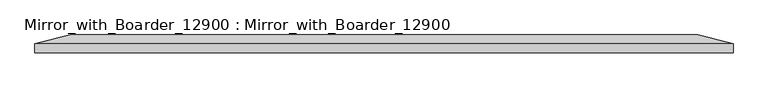
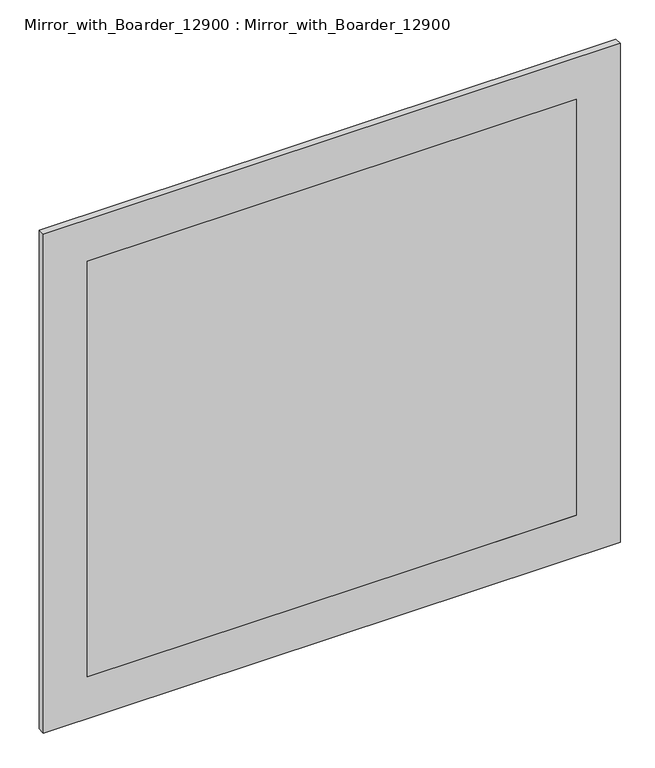
"""IFC4 building model written with IfcOpenShell, lengths in millimetres: proxy geometry, Mirror_with_Boarder_12900 : Mirror_with_Boarder_12900."""

import ifcopenshell
import ifcopenshell.guid

model = None  # the IFC model being written
_history = None  # IfcOwnerHistory: only IFC2X3 demands one
_inside = {}  # id of a spatial element -> (the spatial element, [elements in it])
_under = {}  # id of a project, library or spatial element -> (it, [spatial elements below it])
_declared = {}  # id of a project -> (the project, [libraries it declares])
_typed = {}  # id of a type object -> (the type object, [elements of that type])
_made_of = {}  # id of a material, layer set ... -> (it, [elements and type objects made of it])


def new_model(schema):
    """Start an empty IFC model of exactly this schema.

    Asked for "IFC4X3", IfcOpenShell would pick the latest addendum, in which some entities
    have other attributes; the version numbers below select the first issue.
    IFC2X3 requires an IfcOwnerHistory on every rooted entity: one is made here for all.
    """
    global model, _history
    if schema == "IFC4X3":
        model = ifcopenshell.file(schema_version=(4, 3, 0, 0))
    else:
        model = ifcopenshell.file(schema=schema)
    _inside.clear()
    _under.clear()
    _declared.clear()
    _typed.clear()
    _made_of.clear()
    _history = None
    if model.schema == "IFC2X3":
        org = make("IfcOrganization", Name="unknown")
        user = make(
            "IfcPersonAndOrganization",
            ThePerson=make("IfcPerson", FamilyName="unknown"),
            TheOrganization=org,
        )
        app = make(
            "IfcApplication",
            ApplicationDeveloper=org,
            Version="unknown",
            ApplicationFullName="unknown",
            ApplicationIdentifier="unknown",
        )
        _history = make(
            "IfcOwnerHistory",
            OwningUser=user,
            OwningApplication=app,
            ChangeAction="ADDED",
            CreationDate=0,
        )
    return model


def make(cls, **values):
    """One entity of the class cls with the attributes given. An attribute that is None is left unset."""
    return model.create_entity(
        cls, **{name: value for name, value in values.items() if value is not None}
    )


def rooted(cls, **values):
    """An entity with a GlobalId (a new one), such as an element, a storey or a relation."""
    return make(cls, GlobalId=ifcopenshell.guid.new(), OwnerHistory=_history, **values)


def si_unit(unit_type, name, prefix=None):
    """IfcSIUnit, for example si_unit("LENGTHUNIT", "METRE", prefix="MILLI")."""
    return make("IfcSIUnit", UnitType=unit_type, Prefix=prefix, Name=name)


def assignment(units):
    """IfcUnitAssignment: the units of a project."""
    return None if units is None else make("IfcUnitAssignment", Units=units)


def point(xyz):
    """IfcCartesianPoint."""
    return None if xyz is None else make("IfcCartesianPoint", Coordinates=xyz)


def direction(xyz):
    """IfcDirection."""
    return None if xyz is None else make("IfcDirection", DirectionRatios=xyz)


def frame(location, z_axis=None, x_axis=None):
    """IfcAxis2Placement3D, a coordinate frame: its origin and axes. An axis left out is left unset."""
    return make(
        "IfcAxis2Placement3D",
        Location=point(location),
        Axis=direction(z_axis),
        RefDirection=direction(x_axis),
    )


def origin():
    """The frame at (0, 0, 0) with its axes left unset."""
    return frame((0.0, 0.0, 0.0))


def place(relative_to, where):
    """IfcLocalPlacement: puts the frame where relative to a parent placement (None: the world)."""
    return make(
        "IfcLocalPlacement", PlacementRelTo=relative_to, RelativePlacement=where
    )


def context(
    kind, dimensions, precision=None, world=None, true_north=None, identifier=None
):
    """IfcGeometricRepresentationContext, for example the 3D "Model" context."""
    return make(
        "IfcGeometricRepresentationContext",
        ContextIdentifier=identifier,
        ContextType=kind,
        CoordinateSpaceDimension=dimensions,
        Precision=precision,
        WorldCoordinateSystem=world,
        TrueNorth=true_north,
    )


def project(units=None, contexts=None):
    """IfcProject with its units and contexts."""
    return rooted(
        "IfcProject",
        Name="project",
        RepresentationContexts=contexts,
        UnitsInContext=assignment(units),
    )


def spatial(cls, under=None, at=None, **own):
    """A site, building, storey or space (cls), placed at a placement, below another one or the project."""
    s = rooted(cls, ObjectPlacement=at, **own)
    if under is not None:
        _under.setdefault(under.id(), (under, []))[1].append(s)
    return s


def polyline(points):
    """IfcPolyline through the points."""
    return make("IfcPolyline", Points=[point(p) for p in points])


def outline(outer, holes=None, kind="AREA"):
    """IfcArbitraryClosedProfileDef: a profile drawn as a closed curve; with holes, ...WithVoids."""
    if holes is None:
        return make("IfcArbitraryClosedProfileDef", ProfileType=kind, OuterCurve=outer)
    return make(
        "IfcArbitraryProfileDefWithVoids",
        ProfileType=kind,
        OuterCurve=outer,
        InnerCurves=holes,
    )


def extrude(swept, where, along, depth):
    """IfcExtrudedAreaSolid: the profile swept, set in the frame where, extruded along a direction by depth."""
    return make(
        "IfcExtrudedAreaSolid",
        SweptArea=swept,
        Position=where,
        ExtrudedDirection=direction(along),
        Depth=depth,
    )


def faces_of(points, faces, orient=None, outer=None):
    """IfcFace entities. A face is a list of loops; a loop is a list of indices into points, from 0.

    orient and outer hold one flag for each loop. By default every Orientation is true, the
    first loop of a face is its IfcFaceOuterBound and the others are IfcFaceBound.
    """
    made = []
    for i, loops in enumerate(faces):
        bounds = []
        for j, loop in enumerate(loops):
            is_outer = j == 0 if outer is None else outer[i][j]
            bounds.append(
                make(
                    "IfcFaceOuterBound" if is_outer else "IfcFaceBound",
                    Bound=make("IfcPolyLoop", Polygon=[points[k] for k in loop]),
                    Orientation=True if orient is None else orient[i][j],
                )
            )
        made.append(make("IfcFace", Bounds=bounds))
    return made


def faceted_brep(points, faces, orient=None, outer=None, voids=None):
    """IfcFacetedBrep: a solid bounded by flat faces; with voids (closed shells), ...WithVoids."""
    shared = [point(p) for p in points]
    hull = make("IfcClosedShell", CfsFaces=faces_of(shared, faces, orient, outer))
    if voids is None:
        return make("IfcFacetedBrep", Outer=hull)
    return make(
        "IfcFacetedBrepWithVoids",
        Outer=hull,
        Voids=[
            make(cls, CfsFaces=faces_of(shared, fs, o, b)) for cls, fs, o, b in voids
        ],
    )


def shape(context_of_items, identifier, shape_type, items):
    """IfcShapeRepresentation: the items that make up one representation, for example the "Body"."""
    return make(
        "IfcShapeRepresentation",
        ContextOfItems=context_of_items,
        RepresentationIdentifier=identifier,
        RepresentationType=shape_type,
        Items=items,
    )


def source(mapping_origin, context_of_items, identifier, shape_type, items):
    """IfcRepresentationMap: a shape defined once, which mapped items show again and again."""
    return make(
        "IfcRepresentationMap",
        MappingOrigin=mapping_origin,
        MappedRepresentation=shape(context_of_items, identifier, shape_type, items),
    )


def transform(
    local_origin,
    x_axis=None,
    y_axis=None,
    z_axis=None,
    scale=None,
    scale2=None,
    scale3=None,
    uniform=True,
):
    """IfcCartesianTransformationOperator3D, or its non-uniform kind. x_axis, y_axis, z_axis: its Axis1, 2, 3."""
    if uniform:
        return make(
            "IfcCartesianTransformationOperator3D",
            Axis1=direction(x_axis),
            Axis2=direction(y_axis),
            LocalOrigin=point(local_origin),
            Scale=scale,
            Axis3=direction(z_axis),
        )
    return make(
        "IfcCartesianTransformationOperator3DnonUniform",
        Axis1=direction(x_axis),
        Axis2=direction(y_axis),
        LocalOrigin=point(local_origin),
        Scale=scale,
        Axis3=direction(z_axis),
        Scale2=scale2,
        Scale3=scale3,
    )


def mapped(mapping_source, mapping_target):
    """IfcMappedItem: shows the shape of a source again, moved by a transform."""
    return make(
        "IfcMappedItem", MappingSource=mapping_source, MappingTarget=mapping_target
    )


def made_of(thing, what):
    """Note that an element or type object is made of a material, layer set ...; save() writes the relation."""
    if what is not None:
        _made_of.setdefault(what.id(), (what, []))[1].append(thing)
    return thing


def element(
    cls,
    number,
    at=None,
    inside=None,
    cuts=None,
    type_object=None,
    material=None,
    context=None,
    identifier="Body",
    shape_type=None,
    held_by="IfcProductDefinitionShape",
    body=None,
    shapes=None,
    **own,
):
    """One element of the class cls, such as IfcWall. Its Tag is "e" and its number.

    at: its placement. inside: the storey or other place that contains it. cuts: it is an
    opening in that element (IfcRelVoidsElement). A single representation is given by context,
    identifier, shape_type and body (its items); several are given by shapes. held_by: the class
    of the entity that holds the representations. save() writes the other relations.
    """
    e = rooted(cls, Tag="e%d" % number, ObjectPlacement=at, **own)
    if body is not None:
        shapes = [shape(context, identifier, shape_type, body)]
    if shapes is not None:
        e.Representation = make(held_by, Representations=shapes)
    if inside is not None:
        _inside.setdefault(inside.id(), (inside, []))[1].append(e)
    if cuts is not None:
        rooted(
            "IfcRelVoidsElement", RelatingBuildingElement=cuts, RelatedOpeningElement=e
        )
    if type_object is not None:
        _typed.setdefault(type_object.id(), (type_object, []))[1].append(e)
    return made_of(e, material)


def aggregate(whole, parts):
    """IfcRelAggregates: a whole, such as a stair, and the parts it consists of."""
    return rooted("IfcRelAggregates", RelatingObject=whole, RelatedObjects=parts)


def save(model, path):
    """Write the relations noted so far, then the file.

    IfcRelAggregates (storeys below a building ...), IfcRelContainedInSpatialStructure (elements
    in a storey), IfcRelDefinesByType, IfcRelAssociatesMaterial and IfcRelDeclares: one each for
    every whole, place, type object, material and project.
    """
    for whole, parts in _under.values():
        aggregate(whole, parts)
    for where, things in _inside.values():
        rooted(
            "IfcRelContainedInSpatialStructure",
            RelatedElements=things,
            RelatingStructure=where,
        )
    for kind, things in _typed.values():
        rooted("IfcRelDefinesByType", RelatedObjects=things, RelatingType=kind)
    for what, things in _made_of.values():
        rooted("IfcRelAssociatesMaterial", RelatedObjects=things, RelatingMaterial=what)
    for by, libraries in _declared.values():
        rooted("IfcRelDeclares", RelatingContext=by, RelatedDefinitions=libraries)
    model.write(path)


def mirror_with_boarder_12900_mirror_with_boarder_12900_da111bb4(model_context):
    return source(origin(), model_context, "Body", "SolidModel", [
        faceted_brep([(412.7003906, 63.9960938, 1027.1125), (-412.7003906, 63.9960938, 1027.1125), (-412.7003906, 63.9960938, 1766.8875), (412.7003906, 63.9960938, 1766.8875), (423.8128906, 59.2335938, 1016.0), (423.8128906, 59.2335938, 1778.0), (-423.8128906, 59.2335938, 1778.0), (-423.8128906, 59.2335938, 1016.0), (-423.8128906, 62.4085938, 1016.0), (423.8128906, 62.4085937, 1016.0), (-423.8128906, 62.4085937, 1778.0), (423.8128906, 62.4085937, 1778.0)], [[[0, 1, 2, 3]], [[4, 5, 6, 7]], [[4, 7, 8, 9]], [[7, 6, 10, 8]], [[6, 5, 11, 10]], [[5, 4, 9, 11]], [[8, 1, 0, 9]], [[1, 8, 10, 2]], [[2, 10, 11, 3]], [[9, 0, 3, 11]]]),
        extrude(outline(polyline([(-423.8128906, 59.2335938), (423.8128906, 59.2335938), (423.8128906, 50.8), (-423.8128906, 50.8), (-423.8128906, 59.2335938)])), frame((0.0, 0.0, 1016.0), z_axis=(0.0, 0.0, 1.0), x_axis=(1.0, 0.0, 0.0)), (0.0, 0.0, 1.0), 762.0),
        faceted_brep([(449.2128906, 76.2, 1803.4), (449.2128906, 76.2, 990.6), (-449.2128906, 76.2, 990.6), (-449.2128906, 76.2, 1803.4), (-423.8128906, 76.2, 1778.0), (-423.8128906, 76.2, 1016.0), (423.8128906, 76.2, 1016.0), (423.8128906, 76.2, 1778.0), (-500.0128906, 50.8, 1854.2), (-500.0128906, 50.8, 939.8), (500.0128906, 50.8, 939.8), (500.0128906, 50.8, 1854.2), (-423.8128906, 50.8, 1778.0), (423.8128906, 50.8, 1778.0), (423.8128906, 50.8, 1016.0), (-423.8128906, 50.8, 1016.0), (-423.8128906, 63.9960938, 1778.0), (-423.8128906, 62.4085937, 1778.0), (-423.8128906, 62.4085938, 1016.0), (-423.8128906, 63.9960938, 1016.0), (423.8128906, 62.4085938, 1016.0), (423.8128906, 63.9960938, 1016.0), (423.8128906, 62.4085937, 1778.0), (423.8128906, 63.9960938, 1778.0), (500.0128906, 63.5, 1854.2), (-500.0128906, 63.5, 1854.2), (500.0128906, 63.5, 939.8), (-500.0128906, 63.5, 939.8)], [[[0, 1, 2, 3], [4, 5, 6, 7]], [[8, 9, 10, 11], [12, 13, 14, 15]], [[5, 4, 16, 17, 12, 15, 18, 19]], [[6, 5, 19, 18, 15, 14, 20, 21]], [[7, 6, 21, 20, 14, 13, 22, 23]], [[4, 7, 23, 22, 13, 12, 17, 16]], [[8, 11, 24, 25]], [[11, 10, 26, 24]], [[10, 9, 27, 26]], [[9, 8, 25, 27]], [[26, 1, 0, 24]], [[1, 26, 27, 2]], [[2, 27, 25, 3]], [[24, 0, 3, 25]]]),
    ])


if __name__ == "__main__":
    model = new_model("IFC4")
    model_context = context("Model", 3, world=origin())
    ifc_project = project(units=[si_unit("LENGTHUNIT", "METRE", prefix="MILLI")], contexts=[model_context])
    site = spatial("IfcSite", under=ifc_project)
    building = spatial("IfcBuilding", under=site)
    placement = place(None, origin())
    mirror_with_boarder_12900_mirror_with_boarder_12900_shape = mirror_with_boarder_12900_mirror_with_boarder_12900_da111bb4(model_context)
    element("IfcBuildingElementProxy", 1, Name="Mirror_with_Boarder_12900 : Mirror_with_Boarder_12900", ObjectType="Mirror_with_Boarder_12900 : Mirror_with_Boarder_12900", at=placement, inside=building, context=model_context, shape_type="MappedRepresentation", body=[
        mapped(mirror_with_boarder_12900_mirror_with_boarder_12900_shape, transform((0.0, 0.0, 0.0), x_axis=(1.0, 0.0, 0.0), y_axis=(0.0, 1.0, 0.0), z_axis=(0.0, 0.0, 1.0))),
    ])
    save(model, "model.ifc")

# Revit data of these elements
# Type "Mirror_with_Boarder_12900 : Mirror_with_Boarder_12900"
#   Width = 3' - 3 95/256"
#   Height = 3' - 0"
#   Mirror Frame = Mirror Frame
#   Mirror = Mirror
#   Default Elevation = 0
# Element 1 (IfcBuildingElementProxy, "Mirror_with_Boarder_12900 : Mirror_with_Boarder_12900")
#   Materials on its faces: "Mirror Frame", "Mirror"
# Materials
#   "Mirror Frame": class "Miscellaneous", colour RGB 27 25 23, transparency 0
#   "Mirror": class "Glass", colour RGB 178 191 178, transparency 0, Cost = 0
